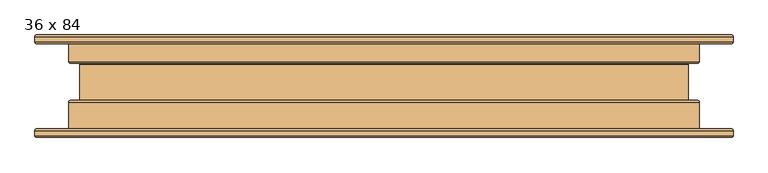
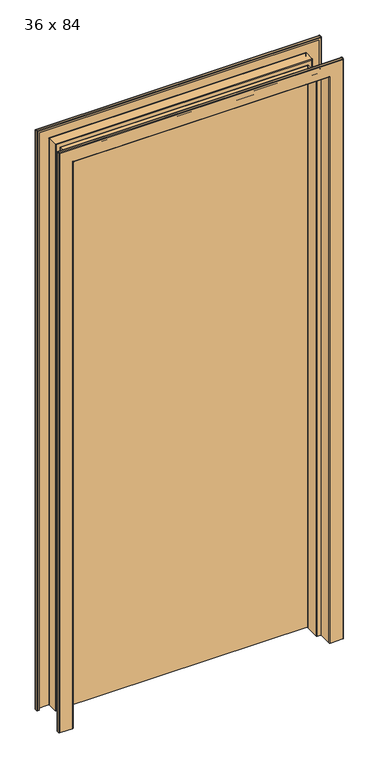
"""IFC4 building model written with IfcOpenShell, lengths in millimetres: door geometry, Door-Dunbarton_Doors-Hollow_Metal_Core : 36 x 84."""

from ifc_helpers import new_model, si_unit, frame, origin, origin_with_axes, place, context, project, spatial, polyline, circle_curve, ellipse_curve, outline, extrude, source, transform, mapped, element, save
from ifc_brep_helpers import plane_surface, cylinder_surface, revolved_surface, advanced_brep


def door_36_x_84_ee10bf19(model_context):
    return source(origin(), model_context, "Body", "SolidModel", [
        advanced_brep(
        [(-505.42825, -61.976, 0.0), (-500.0625, -61.976, 0.0), (-500.0625, -63.53175, 0.0), (-505.42825, -63.53175, 0.0), (-506.44425, -64.54775, 0.0), (-506.44425, -72.0725, 0.0), (-505.42825, -73.0885, 0.0), (-459.77175, -73.0885, 0.0), (-458.75575, -72.0725, 0.0), (-458.75575, -23.27275, 0.0), (-456.184, -20.701, 0.0), (-443.89675, -20.701, 0.0), (-442.88075, -19.685, 0.0), (-442.88075, 32.1056, 0.0), (-443.89675, 33.1216, 0.0), (-456.184, 33.1216, 0.0), (-458.75575, 35.69335, 0.0), (-458.75575, 72.009, 0.0), (-459.77175, 73.025, 0.0), (-505.42825, 73.025, 0.0), (-506.44425, 72.009, 0.0), (-506.44425, 64.48425, 0.0), (-505.42825, 63.46825, 0.0), (-500.0625, 63.46825, 0.0), (-500.0625, 61.9125, 0.0), (-505.42825, 61.9125, 0.0), (-508.0, 64.48425, 0.0), (-508.0, 72.009, 0.0), (-505.42825, 74.58075, 0.0), (-459.77175, 74.58075, 0.0), (-457.2, 72.009, 0.0), (-457.2, 35.69335, 0.0), (-456.184, 34.67735, 0.0), (-443.89675, 34.67735, 0.0), (-441.325, 32.1056, 0.0), (-441.325, -19.685, 0.0), (-443.89675, -22.25675, 0.0), (-456.184, -22.25675, 0.0), (-457.2, -23.27275, 0.0), (-457.2, -72.0725, 0.0), (-459.77175, -74.64425, 0.0), (-505.42825, -74.64425, 0.0), (-508.0, -72.0725, 0.0), (-508.0, -64.54775, 0.0), (-508.0, -64.54775, 2184.4), (-505.42825, -61.976, 2181.82825), (-508.0, -72.0725, 2184.4), (-505.42825, -74.64425, 2181.82825), (-459.77175, -74.64425, 2136.17175), (459.77175, -74.64425, 2136.17175), (459.77175, -74.64425, 0.0), (505.42825, -74.64425, 0.0), (505.42825, -74.64425, 2181.82825), (-457.2, -72.0725, 2133.6), (-457.2, -23.27275, 2133.6), (-456.184, -22.25675, 2132.584), (-443.89675, -22.25675, 2120.29675), (443.89675, -22.25675, 2120.29675), (443.89675, -22.25675, 0.0), (456.184, -22.25675, 0.0), (456.184, -22.25675, 2132.584), (-441.325, -19.685, 2117.725), (-441.325, 32.1056, 2117.725), (-443.89675, 34.67735, 2120.29675), (-456.184, 34.67735, 2132.584), (456.184, 34.67735, 2132.584), (456.184, 34.67735, 0.0), (443.89675, 34.67735, 0.0), (443.89675, 34.67735, 2120.29675), (-457.2, 35.69335, 2133.6), (-457.2, 72.009, 2133.6), (-459.77175, 74.58075, 2136.17175), (-505.42825, 74.58075, 2181.82825), (505.42825, 74.58075, 2181.82825), (505.42825, 74.58075, 0.0), (459.77175, 74.58075, 0.0), (459.77175, 74.58075, 2136.17175), (-508.0, 72.009, 2184.4), (-508.0, 64.48425, 2184.4), (-505.42825, 61.9125, 2181.82825), (-500.0625, 61.9125, 2176.4625), (500.0625, 61.9125, 2176.4625), (500.0625, 61.9125, 0.0), (505.42825, 61.9125, 0.0), (505.42825, 61.9125, 2181.82825), (-500.0625, 63.46825, 2176.4625), (-505.42825, 63.46825, 2181.82825), (505.42825, 63.46825, 2181.82825), (505.42825, 63.46825, 0.0), (500.0625, 63.46825, 0.0), (500.0625, 63.46825, 2176.4625), (-506.44425, 64.48425, 2182.84425), (-506.44425, 72.009, 2182.84425), (-505.42825, 73.025, 2181.82825), (-459.77175, 73.025, 2136.17175), (459.77175, 73.025, 2136.17175), (459.77175, 73.025, 0.0), (505.42825, 73.025, 0.0), (505.42825, 73.025, 2181.82825), (-458.75575, 72.009, 2135.15575), (-458.75575, 35.69335, 2135.15575), (-456.184, 33.1216, 2132.584), (-443.89675, 33.1216, 2120.29675), (443.89675, 33.1216, 2120.29675), (443.89675, 33.1216, 0.0), (456.184, 33.1216, 0.0), (456.184, 33.1216, 2132.584), (-442.88075, 32.1056, 2119.28075), (-442.88075, -19.685, 2119.28075), (-443.89675, -20.701, 2120.29675), (-456.184, -20.701, 2132.584), (456.184, -20.701, 2132.584), (456.184, -20.701, 0.0), (443.89675, -20.701, 0.0), (443.89675, -20.701, 2120.29675), (-458.75575, -23.27275, 2135.15575), (-458.75575, -72.0725, 2135.15575), (-459.77175, -73.0885, 2136.17175), (-505.42825, -73.0885, 2181.82825), (505.42825, -73.0885, 2181.82825), (505.42825, -73.0885, 0.0), (459.77175, -73.0885, 0.0), (459.77175, -73.0885, 2136.17175), (-506.44425, -72.0725, 2182.84425), (-506.44425, -64.54775, 2182.84425), (-505.42825, -63.53175, 2181.82825), (-500.0625, -63.53175, 2176.4625), (500.0625, -63.53175, 2176.4625), (500.0625, -63.53175, 0.0), (505.42825, -63.53175, 0.0), (505.42825, -63.53175, 2181.82825), (-500.0625, -61.976, 2176.4625), (505.42825, -61.976, 2181.82825), (505.42825, -61.976, 0.0), (500.0625, -61.976, 0.0), (500.0625, -61.976, 2176.4625), (508.0, -64.54775, 2184.4), (508.0, -72.0725, 2184.4), (457.2, -72.0725, 2133.6), (457.2, -23.27275, 2133.6), (441.325, -19.685, 2117.725), (441.325, 32.1056, 2117.725), (457.2, 35.69335, 2133.6), (457.2, 72.009, 2133.6), (508.0, 72.009, 2184.4), (508.0, 64.48425, 2184.4), (506.44425, 64.48425, 2182.84425), (506.44425, 72.009, 2182.84425), (458.75575, 72.009, 2135.15575), (458.75575, 35.69335, 2135.15575), (442.88075, 32.1056, 2119.28075), (442.88075, -19.685, 2119.28075), (458.75575, -23.27275, 2135.15575), (458.75575, -72.0725, 2135.15575), (506.44425, -72.0725, 2182.84425), (506.44425, -64.54775, 2182.84425), (508.0, -64.54775, 0.0), (508.0, -72.0725, 0.0), (457.2, -72.0725, 0.0), (457.2, -23.27275, 0.0), (441.325, -19.685, 0.0), (441.325, 32.1056, 0.0), (457.2, 35.69335, 0.0), (457.2, 72.009, 0.0), (508.0, 72.009, 0.0), (508.0, 64.48425, 0.0), (506.44425, 64.48425, 0.0), (506.44425, 72.009, 0.0), (458.75575, 72.009, 0.0), (458.75575, 35.69335, 0.0), (442.88075, 32.1056, 0.0), (442.88075, -19.685, 0.0), (458.75575, -23.27275, 0.0), (458.75575, -72.0725, 0.0), (506.44425, -72.0725, 0.0), (506.44425, -64.54775, 0.0)],
        [
            (0, 1),
            (1, 2),
            (2, 3),
            (3, 4, circle_curve(frame((-505.42825, -64.54775, 0.0), z_axis=(0.0, 0.0, 1.0), x_axis=(0.0, 1.0, 0.0)), 1.016)),
            (4, 5),
            (5, 6, circle_curve(frame((-505.42825, -72.0725, 0.0), z_axis=(0.0, 0.0, 1.0), x_axis=(0.0, 1.0, 0.0)), 1.016)),
            (6, 7),
            (7, 8, circle_curve(frame((-459.77175, -72.0725, 0.0), z_axis=(0.0, 0.0, 1.0), x_axis=(0.0, 1.0, 0.0)), 1.016)),
            (8, 9),
            (9, 10, circle_curve(frame((-456.184, -23.27275, 0.0), z_axis=(0.0, 0.0, -1.0), x_axis=(0.0, 1.0, 0.0)), 2.57175)),
            (10, 11),
            (11, 12, circle_curve(frame((-443.89675, -19.685, 0.0), z_axis=(0.0, 0.0, 1.0), x_axis=(0.0, 1.0, 0.0)), 1.016)),
            (12, 13),
            (13, 14, circle_curve(frame((-443.89675, 32.1056, 0.0), z_axis=(0.0, 0.0, 1.0), x_axis=(0.0, 1.0, 0.0)), 1.016)),
            (14, 15),
            (15, 16, circle_curve(frame((-456.184, 35.69335, 0.0), z_axis=(0.0, 0.0, -1.0), x_axis=(0.0, 1.0, 0.0)), 2.57175)),
            (16, 17),
            (17, 18, circle_curve(frame((-459.77175, 72.009, 0.0), z_axis=(0.0, 0.0, 1.0), x_axis=(0.0, 1.0, 0.0)), 1.016)),
            (18, 19),
            (19, 20, circle_curve(frame((-505.42825, 72.009, 0.0), z_axis=(0.0, 0.0, 1.0), x_axis=(0.0, 1.0, 0.0)), 1.016)),
            (20, 21),
            (21, 22, circle_curve(frame((-505.42825, 64.48425, 0.0), z_axis=(0.0, 0.0, 1.0), x_axis=(0.0, 1.0, 0.0)), 1.016)),
            (22, 23),
            (23, 24),
            (24, 25),
            (25, 26, circle_curve(frame((-505.42825, 64.48425, 0.0), z_axis=(0.0, 0.0, -1.0), x_axis=(0.0, 1.0, 0.0)), 2.57175)),
            (26, 27),
            (27, 28, circle_curve(frame((-505.42825, 72.009, 0.0), z_axis=(0.0, 0.0, -1.0), x_axis=(0.0, 1.0, 0.0)), 2.57175)),
            (28, 29),
            (29, 30, circle_curve(frame((-459.77175, 72.009, 0.0), z_axis=(0.0, 0.0, -1.0), x_axis=(0.0, 1.0, 0.0)), 2.57175)),
            (30, 31),
            (31, 32, circle_curve(frame((-456.184, 35.69335, 0.0), z_axis=(0.0, 0.0, 1.0), x_axis=(0.0, 1.0, 0.0)), 1.016)),
            (32, 33),
            (33, 34, circle_curve(frame((-443.89675, 32.1056, 0.0), z_axis=(0.0, 0.0, -1.0), x_axis=(0.0, 1.0, 0.0)), 2.57175)),
            (34, 35),
            (35, 36, circle_curve(frame((-443.89675, -19.685, 0.0), z_axis=(0.0, 0.0, -1.0), x_axis=(0.0, 1.0, 0.0)), 2.57175)),
            (36, 37),
            (37, 38, circle_curve(frame((-456.184, -23.27275, 0.0), z_axis=(0.0, 0.0, 1.0), x_axis=(0.0, 1.0, 0.0)), 1.016)),
            (38, 39),
            (39, 40, circle_curve(frame((-459.77175, -72.0725, 0.0), z_axis=(0.0, 0.0, -1.0), x_axis=(0.0, 1.0, 0.0)), 2.57175)),
            (40, 41),
            (41, 42, circle_curve(frame((-505.42825, -72.0725, 0.0), z_axis=(0.0, 0.0, -1.0), x_axis=(0.0, 1.0, 0.0)), 2.57175)),
            (42, 43),
            (43, 0, circle_curve(frame((-505.42825, -64.54775, 0.0), z_axis=(0.0, 0.0, -1.0), x_axis=(0.0, 1.0, 0.0)), 2.57175)),
            (43, 44),
            (44, 45, ellipse_curve(frame((-505.42825, -64.54775, 2181.82825), z_axis=(-0.7071067811865475, 0.0, -0.7071067811865475), x_axis=(0.7071067811865474, 0.0, -0.7071067811865476)), 3.6370037, 2.57175)),
            (45, 0),
            (42, 46),
            (46, 44),
            (41, 47),
            (47, 46, ellipse_curve(frame((-505.42825, -72.0725, 2181.82825), z_axis=(-0.7071067811865475, 0.0, -0.7071067811865475), x_axis=(0.7071067811865474, 0.0, -0.7071067811865476)), 3.6370037, 2.57175)),
            (40, 48),
            (48, 49),
            (49, 50),
            (50, 51),
            (51, 52),
            (52, 47),
            (39, 53),
            (53, 48, ellipse_curve(frame((-459.77175, -72.0725, 2136.17175), z_axis=(-0.7071067811865475, 0.0, -0.7071067811865475), x_axis=(0.7071067811865474, 0.0, -0.7071067811865476)), 3.6370037, 2.57175)),
            (38, 54),
            (54, 53),
            (37, 55),
            (55, 54, ellipse_curve(frame((-456.184, -23.27275, 2132.584), z_axis=(0.7071067811865475, 0.0, 0.7071067811865475), x_axis=(-0.7071067811865474, 0.0, 0.7071067811865476)), 1.436841, 1.016)),
            (36, 56),
            (56, 57),
            (57, 58),
            (58, 59),
            (59, 60),
            (60, 55),
            (35, 61),
            (61, 56, ellipse_curve(frame((-443.89675, -19.685, 2120.29675), z_axis=(-0.7071067811865475, 0.0, -0.7071067811865475), x_axis=(0.7071067811865474, 0.0, -0.7071067811865476)), 3.6370037, 2.57175)),
            (34, 62),
            (62, 61),
            (33, 63),
            (63, 62, ellipse_curve(frame((-443.89675, 32.1056, 2120.29675), z_axis=(-0.7071067811865475, 0.0, -0.7071067811865475), x_axis=(0.7071067811865474, 0.0, -0.7071067811865476)), 3.6370037, 2.57175)),
            (32, 64),
            (64, 65),
            (65, 66),
            (66, 67),
            (67, 68),
            (68, 63),
            (31, 69),
            (69, 64, ellipse_curve(frame((-456.184, 35.69335, 2132.584), z_axis=(0.7071067811865475, 0.0, 0.7071067811865475), x_axis=(-0.7071067811865474, 0.0, 0.7071067811865476)), 1.436841, 1.016)),
            (30, 70),
            (70, 69),
            (29, 71),
            (71, 70, ellipse_curve(frame((-459.77175, 72.009, 2136.17175), z_axis=(-0.7071067811865475, 0.0, -0.7071067811865475), x_axis=(0.7071067811865474, 0.0, -0.7071067811865476)), 3.6370037, 2.57175)),
            (28, 72),
            (72, 73),
            (73, 74),
            (74, 75),
            (75, 76),
            (76, 71),
            (27, 77),
            (77, 72, ellipse_curve(frame((-505.42825, 72.009, 2181.82825), z_axis=(-0.7071067811865475, 0.0, -0.7071067811865475), x_axis=(0.7071067811865474, 0.0, -0.7071067811865476)), 3.6370037, 2.57175)),
            (26, 78),
            (78, 77),
            (25, 79),
            (79, 78, ellipse_curve(frame((-505.42825, 64.48425, 2181.82825), z_axis=(-0.7071067811865475, 0.0, -0.7071067811865475), x_axis=(0.7071067811865474, 0.0, -0.7071067811865476)), 3.6370037, 2.57175)),
            (24, 80),
            (80, 81),
            (81, 82),
            (82, 83),
            (83, 84),
            (84, 79),
            (23, 85),
            (85, 80),
            (22, 86),
            (86, 87),
            (87, 88),
            (88, 89),
            (89, 90),
            (90, 85),
            (21, 91),
            (91, 86, ellipse_curve(frame((-505.42825, 64.48425, 2181.82825), z_axis=(0.7071067811865475, 0.0, 0.7071067811865475), x_axis=(-0.7071067811865474, 0.0, 0.7071067811865476)), 1.436841, 1.016)),
            (20, 92),
            (92, 91),
            (19, 93),
            (93, 92, ellipse_curve(frame((-505.42825, 72.009, 2181.82825), z_axis=(0.7071067811865475, 0.0, 0.7071067811865475), x_axis=(-0.7071067811865474, 0.0, 0.7071067811865476)), 1.436841, 1.016)),
            (18, 94),
            (94, 95),
            (95, 96),
            (96, 97),
            (97, 98),
            (98, 93),
            (17, 99),
            (99, 94, ellipse_curve(frame((-459.77175, 72.009, 2136.17175), z_axis=(0.7071067811865475, 0.0, 0.7071067811865475), x_axis=(-0.7071067811865474, 0.0, 0.7071067811865476)), 1.436841, 1.016)),
            (16, 100),
            (100, 99),
            (15, 101),
            (101, 100, ellipse_curve(frame((-456.184, 35.69335, 2132.584), z_axis=(-0.7071067811865475, 0.0, -0.7071067811865475), x_axis=(0.7071067811865474, 0.0, -0.7071067811865476)), 3.6370037, 2.57175)),
            (14, 102),
            (102, 103),
            (103, 104),
            (104, 105),
            (105, 106),
            (106, 101),
            (13, 107),
            (107, 102, ellipse_curve(frame((-443.89675, 32.1056, 2120.29675), z_axis=(0.7071067811865475, 0.0, 0.7071067811865475), x_axis=(-0.7071067811865474, 0.0, 0.7071067811865476)), 1.436841, 1.016)),
            (12, 108),
            (108, 107),
            (11, 109),
            (109, 108, ellipse_curve(frame((-443.89675, -19.685, 2120.29675), z_axis=(0.7071067811865475, 0.0, 0.7071067811865475), x_axis=(-0.7071067811865474, 0.0, 0.7071067811865476)), 1.436841, 1.016)),
            (10, 110),
            (110, 111),
            (111, 112),
            (112, 113),
            (113, 114),
            (114, 109),
            (9, 115),
            (115, 110, ellipse_curve(frame((-456.184, -23.27275, 2132.584), z_axis=(-0.7071067811865475, 0.0, -0.7071067811865475), x_axis=(0.7071067811865474, 0.0, -0.7071067811865476)), 3.6370037, 2.57175)),
            (8, 116),
            (116, 115),
            (7, 117),
            (117, 116, ellipse_curve(frame((-459.77175, -72.0725, 2136.17175), z_axis=(0.7071067811865475, 0.0, 0.7071067811865475), x_axis=(-0.7071067811865474, 0.0, 0.7071067811865476)), 1.436841, 1.016)),
            (6, 118),
            (118, 119),
            (119, 120),
            (120, 121),
            (121, 122),
            (122, 117),
            (5, 123),
            (123, 118, ellipse_curve(frame((-505.42825, -72.0725, 2181.82825), z_axis=(0.7071067811865475, 0.0, 0.7071067811865475), x_axis=(-0.7071067811865474, 0.0, 0.7071067811865476)), 1.436841, 1.016)),
            (4, 124),
            (124, 123),
            (3, 125),
            (125, 124, ellipse_curve(frame((-505.42825, -64.54775, 2181.82825), z_axis=(0.7071067811865475, 0.0, 0.7071067811865475), x_axis=(-0.7071067811865474, 0.0, 0.7071067811865476)), 1.436841, 1.016)),
            (2, 126),
            (126, 127),
            (127, 128),
            (128, 129),
            (129, 130),
            (130, 125),
            (1, 131),
            (131, 126),
            (45, 132),
            (132, 133),
            (133, 134),
            (134, 135),
            (135, 131),
            (44, 136),
            (136, 132, ellipse_curve(frame((505.42825, -64.54775, 2181.82825), z_axis=(-0.7071067811865475, 0.0, 0.7071067811865475), x_axis=(-0.7071067811865476, 0.0, -0.7071067811865474)), 3.6370037, 2.57175)),
            (46, 137),
            (137, 136),
            (52, 137, ellipse_curve(frame((505.42825, -72.0725, 2181.82825), z_axis=(-0.7071067811865475, 0.0, 0.7071067811865475), x_axis=(-0.7071067811865476, 0.0, -0.7071067811865474)), 3.6370037, 2.57175)),
            (53, 138),
            (138, 49, ellipse_curve(frame((459.77175, -72.0725, 2136.17175), z_axis=(-0.7071067811865475, 0.0, 0.7071067811865475), x_axis=(-0.7071067811865476, 0.0, -0.7071067811865474)), 3.6370037, 2.57175)),
            (54, 139),
            (139, 138),
            (60, 139, ellipse_curve(frame((456.184, -23.27275, 2132.584), z_axis=(0.7071067811865475, 0.0, -0.7071067811865475), x_axis=(0.7071067811865476, 0.0, 0.7071067811865474)), 1.436841, 1.016)),
            (61, 140),
            (140, 57, ellipse_curve(frame((443.89675, -19.685, 2120.29675), z_axis=(-0.7071067811865475, 0.0, 0.7071067811865475), x_axis=(-0.7071067811865476, 0.0, -0.7071067811865474)), 3.6370037, 2.57175)),
            (62, 141),
            (141, 140),
            (68, 141, ellipse_curve(frame((443.89675, 32.1056, 2120.29675), z_axis=(-0.7071067811865475, 0.0, 0.7071067811865475), x_axis=(-0.7071067811865476, 0.0, -0.7071067811865474)), 3.6370037, 2.57175)),
            (69, 142),
            (142, 65, ellipse_curve(frame((456.184, 35.69335, 2132.584), z_axis=(0.7071067811865475, 0.0, -0.7071067811865475), x_axis=(0.7071067811865476, 0.0, 0.7071067811865474)), 1.436841, 1.016)),
            (70, 143),
            (143, 142),
            (76, 143, ellipse_curve(frame((459.77175, 72.009, 2136.17175), z_axis=(-0.7071067811865475, 0.0, 0.7071067811865475), x_axis=(-0.7071067811865476, 0.0, -0.7071067811865474)), 3.6370037, 2.57175)),
            (77, 144),
            (144, 73, ellipse_curve(frame((505.42825, 72.009, 2181.82825), z_axis=(-0.7071067811865475, 0.0, 0.7071067811865475), x_axis=(-0.7071067811865476, 0.0, -0.7071067811865474)), 3.6370037, 2.57175)),
            (78, 145),
            (145, 144),
            (84, 145, ellipse_curve(frame((505.42825, 64.48425, 2181.82825), z_axis=(-0.7071067811865475, 0.0, 0.7071067811865475), x_axis=(-0.7071067811865476, 0.0, -0.7071067811865474)), 3.6370037, 2.57175)),
            (90, 81),
            (91, 146),
            (146, 87, ellipse_curve(frame((505.42825, 64.48425, 2181.82825), z_axis=(0.7071067811865475, 0.0, -0.7071067811865475), x_axis=(0.7071067811865476, 0.0, 0.7071067811865474)), 1.436841, 1.016)),
            (92, 147),
            (147, 146),
            (98, 147, ellipse_curve(frame((505.42825, 72.009, 2181.82825), z_axis=(0.7071067811865475, 0.0, -0.7071067811865475), x_axis=(0.7071067811865476, 0.0, 0.7071067811865474)), 1.436841, 1.016)),
            (99, 148),
            (148, 95, ellipse_curve(frame((459.77175, 72.009, 2136.17175), z_axis=(0.7071067811865475, 0.0, -0.7071067811865475), x_axis=(0.7071067811865476, 0.0, 0.7071067811865474)), 1.436841, 1.016)),
            (100, 149),
            (149, 148),
            (106, 149, ellipse_curve(frame((456.184, 35.69335, 2132.584), z_axis=(-0.7071067811865475, 0.0, 0.7071067811865475), x_axis=(-0.7071067811865476, 0.0, -0.7071067811865474)), 3.6370037, 2.57175)),
            (107, 150),
            (150, 103, ellipse_curve(frame((443.89675, 32.1056, 2120.29675), z_axis=(0.7071067811865475, 0.0, -0.7071067811865475), x_axis=(0.7071067811865476, 0.0, 0.7071067811865474)), 1.436841, 1.016)),
            (108, 151),
            (151, 150),
            (114, 151, ellipse_curve(frame((443.89675, -19.685, 2120.29675), z_axis=(0.7071067811865475, 0.0, -0.7071067811865475), x_axis=(0.7071067811865476, 0.0, 0.7071067811865474)), 1.436841, 1.016)),
            (115, 152),
            (152, 111, ellipse_curve(frame((456.184, -23.27275, 2132.584), z_axis=(-0.7071067811865475, 0.0, 0.7071067811865475), x_axis=(-0.7071067811865476, 0.0, -0.7071067811865474)), 3.6370037, 2.57175)),
            (116, 153),
            (153, 152),
            (122, 153, ellipse_curve(frame((459.77175, -72.0725, 2136.17175), z_axis=(0.7071067811865475, 0.0, -0.7071067811865475), x_axis=(0.7071067811865476, 0.0, 0.7071067811865474)), 1.436841, 1.016)),
            (123, 154),
            (154, 119, ellipse_curve(frame((505.42825, -72.0725, 2181.82825), z_axis=(0.7071067811865475, 0.0, -0.7071067811865475), x_axis=(0.7071067811865476, 0.0, 0.7071067811865474)), 1.436841, 1.016)),
            (124, 155),
            (155, 154),
            (130, 155, ellipse_curve(frame((505.42825, -64.54775, 2181.82825), z_axis=(0.7071067811865475, 0.0, -0.7071067811865475), x_axis=(0.7071067811865476, 0.0, 0.7071067811865474)), 1.436841, 1.016)),
            (135, 127),
            (133, 156, circle_curve(frame((505.42825, -64.54775, 0.0), z_axis=(0.0, 0.0, -1.0), x_axis=(0.0, 1.0, 0.0)), 2.57175)),
            (156, 157),
            (157, 51, circle_curve(frame((505.42825, -72.0725, 0.0), z_axis=(0.0, 0.0, -1.0), x_axis=(0.0, 1.0, 0.0)), 2.57175)),
            (50, 158, circle_curve(frame((459.77175, -72.0725, 0.0), z_axis=(0.0, 0.0, -1.0), x_axis=(0.0, 1.0, 0.0)), 2.57175)),
            (158, 159),
            (159, 59, circle_curve(frame((456.184, -23.27275, 0.0), z_axis=(0.0, 0.0, 1.0), x_axis=(0.0, 1.0, 0.0)), 1.016)),
            (58, 160, circle_curve(frame((443.89675, -19.685, 0.0), z_axis=(0.0, 0.0, -1.0), x_axis=(0.0, 1.0, 0.0)), 2.57175)),
            (160, 161),
            (161, 67, circle_curve(frame((443.89675, 32.1056, 0.0), z_axis=(0.0, 0.0, -1.0), x_axis=(0.0, 1.0, 0.0)), 2.57175)),
            (66, 162, circle_curve(frame((456.184, 35.69335, 0.0), z_axis=(0.0, 0.0, 1.0), x_axis=(0.0, 1.0, 0.0)), 1.016)),
            (162, 163),
            (163, 75, circle_curve(frame((459.77175, 72.009, 0.0), z_axis=(0.0, 0.0, -1.0), x_axis=(0.0, 1.0, 0.0)), 2.57175)),
            (74, 164, circle_curve(frame((505.42825, 72.009, 0.0), z_axis=(0.0, 0.0, -1.0), x_axis=(0.0, 1.0, 0.0)), 2.57175)),
            (164, 165),
            (165, 83, circle_curve(frame((505.42825, 64.48425, 0.0), z_axis=(0.0, 0.0, -1.0), x_axis=(0.0, 1.0, 0.0)), 2.57175)),
            (82, 89),
            (88, 166, circle_curve(frame((505.42825, 64.48425, 0.0), z_axis=(0.0, 0.0, 1.0), x_axis=(0.0, 1.0, 0.0)), 1.016)),
            (166, 167),
            (167, 97, circle_curve(frame((505.42825, 72.009, 0.0), z_axis=(0.0, 0.0, 1.0), x_axis=(0.0, 1.0, 0.0)), 1.016)),
            (96, 168, circle_curve(frame((459.77175, 72.009, 0.0), z_axis=(0.0, 0.0, 1.0), x_axis=(0.0, 1.0, 0.0)), 1.016)),
            (168, 169),
            (169, 105, circle_curve(frame((456.184, 35.69335, 0.0), z_axis=(0.0, 0.0, -1.0), x_axis=(0.0, 1.0, 0.0)), 2.57175)),
            (104, 170, circle_curve(frame((443.89675, 32.1056, 0.0), z_axis=(0.0, 0.0, 1.0), x_axis=(0.0, 1.0, 0.0)), 1.016)),
            (170, 171),
            (171, 113, circle_curve(frame((443.89675, -19.685, 0.0), z_axis=(0.0, 0.0, 1.0), x_axis=(0.0, 1.0, 0.0)), 1.016)),
            (112, 172, circle_curve(frame((456.184, -23.27275, 0.0), z_axis=(0.0, 0.0, -1.0), x_axis=(0.0, 1.0, 0.0)), 2.57175)),
            (172, 173),
            (173, 121, circle_curve(frame((459.77175, -72.0725, 0.0), z_axis=(0.0, 0.0, 1.0), x_axis=(0.0, 1.0, 0.0)), 1.016)),
            (120, 174, circle_curve(frame((505.42825, -72.0725, 0.0), z_axis=(0.0, 0.0, 1.0), x_axis=(0.0, 1.0, 0.0)), 1.016)),
            (174, 175),
            (175, 129, circle_curve(frame((505.42825, -64.54775, 0.0), z_axis=(0.0, 0.0, 1.0), x_axis=(0.0, 1.0, 0.0)), 1.016)),
            (128, 134),
            (136, 156),
            (137, 157),
            (138, 158),
            (139, 159),
            (140, 160),
            (141, 161),
            (142, 162),
            (143, 163),
            (144, 164),
            (145, 165),
            (146, 166),
            (147, 167),
            (148, 168),
            (149, 169),
            (150, 170),
            (151, 171),
            (152, 172),
            (153, 173),
            (154, 174),
            (155, 175),
        ],
        [
            plane_surface(frame((-468.3125, 61.9125, 0.0), z_axis=(0.0, 0.0, -1.0), x_axis=(1.0, 0.0, 0.0))),
            cylinder_surface(frame((-505.42825, -64.54775, 0.0), z_axis=(0.0, 0.0, -1.0), x_axis=(0.0, 1.0, 0.0)), 2.57175),
            plane_surface(frame((-508.0, -64.54775, 0.0), z_axis=(-1.0, 0.0, 0.0), x_axis=(0.0, 0.0, 1.0))),
            cylinder_surface(frame((-505.42825, -72.0725, 0.0), z_axis=(0.0, 0.0, -1.0), x_axis=(0.0, 1.0, 0.0)), 2.57175),
            plane_surface(frame((-505.42825, -74.64425, 0.0), z_axis=(0.0, -1.0, 0.0), x_axis=(0.0, 0.0, 1.0))),
            cylinder_surface(frame((-459.77175, -72.0725, 0.0), z_axis=(0.0, 0.0, -1.0), x_axis=(0.0, 1.0, 0.0)), 2.57175),
            plane_surface(frame((-457.2, -72.0725, 0.0), z_axis=(1.0, 0.0, 0.0), x_axis=(0.0, 0.0, 1.0))),
            revolved_surface(polyline([(-456.184, -22.256749999999997, 2133.600000014587), (-456.184, -22.256749999999997, 0.0)]), (-456.184, -23.27275, 0.0), (0.0, 0.0, 1.0)),
            plane_surface(frame((-456.184, -22.25675, 0.0), z_axis=(0.0, -1.0, 0.0), x_axis=(0.0, 0.0, 1.0))),
            cylinder_surface(frame((-443.89675, -19.685, 0.0), z_axis=(0.0, 0.0, -1.0), x_axis=(0.0, 1.0, 0.0)), 2.57175),
            plane_surface(frame((-441.325, -19.685, 0.0), z_axis=(1.0, 0.0, 0.0), x_axis=(0.0, 0.0, 1.0))),
            cylinder_surface(frame((-443.89675, 32.1056, 0.0), z_axis=(0.0, 0.0, -1.0), x_axis=(0.0, 1.0, 0.0)), 2.57175),
            plane_surface(frame((-443.89675, 34.67735, 0.0), z_axis=(0.0, 1.0, 0.0), x_axis=(0.0, 0.0, 1.0))),
            revolved_surface(polyline([(-456.184, 36.70935, 2133.600000014587), (-456.184, 36.70935, 0.0)]), (-456.184, 35.69335, 0.0), (0.0, 0.0, 1.0)),
            plane_surface(frame((-457.2, 35.69335, 0.0), z_axis=(1.0, 0.0, 0.0), x_axis=(0.0, 0.0, 1.0))),
            cylinder_surface(frame((-459.77175, 72.009, 0.0), z_axis=(0.0, 0.0, -1.0), x_axis=(0.0, 1.0, 0.0)), 2.57175),
            plane_surface(frame((-459.77175, 74.58075, 0.0), z_axis=(0.0, 1.0, 0.0), x_axis=(0.0, 0.0, 1.0))),
            cylinder_surface(frame((-505.42825, 72.009, 0.0), z_axis=(0.0, 0.0, -1.0), x_axis=(0.0, 1.0, 0.0)), 2.57175),
            plane_surface(frame((-508.0, 72.009, 0.0), z_axis=(-1.0, 0.0, 0.0), x_axis=(0.0, 0.0, 1.0))),
            cylinder_surface(frame((-505.42825, 64.48425, 0.0), z_axis=(0.0, 0.0, -1.0), x_axis=(0.0, 1.0, 0.0)), 2.57175),
            plane_surface(frame((-505.42825, 61.9125, 0.0), z_axis=(0.0, -1.0, 0.0), x_axis=(0.0, 0.0, 1.0))),
            plane_surface(frame((-500.0625, 61.9125, 0.0), z_axis=(1.0, 0.0, 0.0), x_axis=(0.0, 0.0, 1.0))),
            plane_surface(frame((-500.0625, 63.46825, 0.0), z_axis=(0.0, 1.0, 0.0), x_axis=(0.0, 0.0, 1.0))),
            revolved_surface(polyline([(-505.42825, 65.50025000000001, 2182.844250014587), (-505.42825, 65.50025000000001, 0.0)]), (-505.42825, 64.48425, 0.0), (0.0, 0.0, 1.0)),
            plane_surface(frame((-506.44425, 64.48425, 0.0), z_axis=(1.0, 0.0, 0.0), x_axis=(0.0, 0.0, 1.0))),
            revolved_surface(polyline([(-505.42825, 73.025, 2182.844250014587), (-505.42825, 73.025, 0.0)]), (-505.42825, 72.009, 0.0), (0.0, 0.0, 1.0)),
            plane_surface(frame((-505.42825, 73.025, 0.0), z_axis=(0.0, -1.0, 0.0), x_axis=(0.0, 0.0, 1.0))),
            revolved_surface(polyline([(-459.77175, 73.025, 2137.187750014587), (-459.77175, 73.025, 0.0)]), (-459.77175, 72.009, 0.0), (0.0, 0.0, 1.0)),
            plane_surface(frame((-458.75575, 72.009, 0.0), z_axis=(-1.0, 0.0, 0.0), x_axis=(0.0, 0.0, 1.0))),
            cylinder_surface(frame((-456.184, 35.69335, 0.0), z_axis=(0.0, 0.0, -1.0), x_axis=(0.0, 1.0, 0.0)), 2.57175),
            plane_surface(frame((-456.184, 33.1216, 0.0), z_axis=(0.0, -1.0, 0.0), x_axis=(0.0, 0.0, 1.0))),
            revolved_surface(polyline([(-443.89675, 33.1216, 2121.312750014587), (-443.89675, 33.1216, 0.0)]), (-443.89675, 32.1056, 0.0), (0.0, 0.0, 1.0)),
            plane_surface(frame((-442.88075, 32.1056, 0.0), z_axis=(-1.0, 0.0, 0.0), x_axis=(0.0, 0.0, 1.0))),
            revolved_surface(polyline([(-443.89675, -18.668999999999997, 2121.312750014587), (-443.89675, -18.668999999999997, 0.0)]), (-443.89675, -19.685, 0.0), (0.0, 0.0, 1.0)),
            plane_surface(frame((-443.89675, -20.701, 0.0), z_axis=(0.0, 1.0, 0.0), x_axis=(0.0, 0.0, 1.0))),
            cylinder_surface(frame((-456.184, -23.27275, 0.0), z_axis=(0.0, 0.0, -1.0), x_axis=(0.0, 1.0, 0.0)), 2.57175),
            plane_surface(frame((-458.75575, -23.27275, 0.0), z_axis=(-1.0, 0.0, 0.0), x_axis=(0.0, 0.0, 1.0))),
            revolved_surface(polyline([(-459.77175, -71.0565, 2137.187750014587), (-459.77175, -71.0565, 0.0)]), (-459.77175, -72.0725, 0.0), (0.0, 0.0, 1.0)),
            plane_surface(frame((-459.77175, -73.0885, 0.0), z_axis=(0.0, 1.0, 0.0), x_axis=(0.0, 0.0, 1.0))),
            revolved_surface(polyline([(-505.42825, -71.0565, 2182.844250014587), (-505.42825, -71.0565, 0.0)]), (-505.42825, -72.0725, 0.0), (0.0, 0.0, 1.0)),
            plane_surface(frame((-506.44425, -72.0725, 0.0), z_axis=(1.0, 0.0, 0.0), x_axis=(0.0, 0.0, 1.0))),
            revolved_surface(polyline([(-505.42825, -63.531749999999995, 2182.844250014587), (-505.42825, -63.531749999999995, 0.0)]), (-505.42825, -64.54775, 0.0), (0.0, 0.0, 1.0)),
            plane_surface(frame((-505.42825, -63.53175, 0.0), z_axis=(0.0, -1.0, 0.0), x_axis=(0.0, 0.0, 1.0))),
            plane_surface(frame((-500.0625, -63.53175, 0.0), z_axis=(1.0, 0.0, 0.0), x_axis=(0.0, 0.0, 1.0))),
            plane_surface(frame((-500.0625, -61.976, 0.0), z_axis=(0.0, 1.0, 0.0), x_axis=(0.0, 0.0, 1.0))),
            cylinder_surface(frame((-468.3125, -64.54775, 2181.82825), z_axis=(-1.0, 0.0, 0.0), x_axis=(0.0, 1.0, 0.0)), 2.57175),
            plane_surface(frame((-508.0, -64.54775, 2184.4), z_axis=(0.0, 0.0, 1.0), x_axis=(1.0, 0.0, 0.0))),
            cylinder_surface(frame((-468.3125, -72.0725, 2181.82825), z_axis=(-1.0, 0.0, 0.0), x_axis=(0.0, 1.0, 0.0)), 2.57175),
            cylinder_surface(frame((-468.3125, -72.0725, 2136.17175), z_axis=(-1.0, 0.0, 0.0), x_axis=(0.0, 1.0, 0.0)), 2.57175),
            plane_surface(frame((-457.2, -72.0725, 2133.6), z_axis=(0.0, 0.0, -1.0), x_axis=(1.0, 0.0, 0.0))),
            revolved_surface(polyline([(457.20000001458686, -22.256749999999997, 2132.584), (-457.20000001458686, -22.256749999999997, 2132.584)]), (-468.3125, -23.27275, 2132.584), (1.0, 0.0, 0.0)),
            cylinder_surface(frame((-468.3125, -19.685, 2120.29675), z_axis=(-1.0, 0.0, 0.0), x_axis=(0.0, 1.0, 0.0)), 2.57175),
            plane_surface(frame((-441.325, -19.685, 2117.725), z_axis=(0.0, 0.0, -1.0), x_axis=(1.0, 0.0, 0.0))),
            cylinder_surface(frame((-468.3125, 32.1056, 2120.29675), z_axis=(-1.0, 0.0, 0.0), x_axis=(0.0, 1.0, 0.0)), 2.57175),
            revolved_surface(polyline([(457.20000001458686, 36.70935, 2132.584), (-457.20000001458686, 36.70935, 2132.584)]), (-468.3125, 35.69335, 2132.584), (1.0, 0.0, 0.0)),
            plane_surface(frame((-457.2, 35.69335, 2133.6), z_axis=(0.0, 0.0, -1.0), x_axis=(1.0, 0.0, 0.0))),
            cylinder_surface(frame((-468.3125, 72.009, 2136.17175), z_axis=(-1.0, 0.0, 0.0), x_axis=(0.0, 1.0, 0.0)), 2.57175),
            cylinder_surface(frame((-468.3125, 72.009, 2181.82825), z_axis=(-1.0, 0.0, 0.0), x_axis=(0.0, 1.0, 0.0)), 2.57175),
            plane_surface(frame((-508.0, 72.009, 2184.4), z_axis=(0.0, 0.0, 1.0), x_axis=(1.0, 0.0, 0.0))),
            cylinder_surface(frame((-468.3125, 64.48425, 2181.82825), z_axis=(-1.0, 0.0, 0.0), x_axis=(0.0, 1.0, 0.0)), 2.57175),
            plane_surface(frame((-500.0625, 61.9125, 2176.4625), z_axis=(0.0, 0.0, -1.0), x_axis=(1.0, 0.0, 0.0))),
            revolved_surface(polyline([(506.4442500145868, 65.50025000000001, 2181.82825), (-506.4442500145868, 65.50025000000001, 2181.82825)]), (-468.3125, 64.48425, 2181.82825), (1.0, 0.0, 0.0)),
            plane_surface(frame((-506.44425, 64.48425, 2182.84425), z_axis=(0.0, 0.0, -1.0), x_axis=(1.0, 0.0, 0.0))),
            revolved_surface(polyline([(506.4442500145868, 73.025, 2181.82825), (-506.4442500145868, 73.025, 2181.82825)]), (-468.3125, 72.009, 2181.82825), (1.0, 0.0, 0.0)),
            revolved_surface(polyline([(460.7877500145869, 73.025, 2136.17175), (-460.78775001458683, 73.025, 2136.17175)]), (-468.3125, 72.009, 2136.17175), (1.0, 0.0, 0.0)),
            plane_surface(frame((-458.75575, 72.009, 2135.15575), z_axis=(0.0, 0.0, 1.0), x_axis=(1.0, 0.0, 0.0))),
            cylinder_surface(frame((-468.3125, 35.69335, 2132.584), z_axis=(-1.0, 0.0, 0.0), x_axis=(0.0, 1.0, 0.0)), 2.57175),
            revolved_surface(polyline([(444.9127500145869, 33.1216, 2120.29675), (-444.91275001458683, 33.1216, 2120.29675)]), (-468.3125, 32.1056, 2120.29675), (1.0, 0.0, 0.0)),
            plane_surface(frame((-442.88075, 32.1056, 2119.28075), z_axis=(0.0, 0.0, 1.0), x_axis=(1.0, 0.0, 0.0))),
            revolved_surface(polyline([(444.9127500145869, -18.668999999999997, 2120.29675), (-444.91275001458683, -18.668999999999997, 2120.29675)]), (-468.3125, -19.685, 2120.29675), (1.0, 0.0, 0.0)),
            cylinder_surface(frame((-468.3125, -23.27275, 2132.584), z_axis=(-1.0, 0.0, 0.0), x_axis=(0.0, 1.0, 0.0)), 2.57175),
            plane_surface(frame((-458.75575, -23.27275, 2135.15575), z_axis=(0.0, 0.0, 1.0), x_axis=(1.0, 0.0, 0.0))),
            revolved_surface(polyline([(460.7877500145869, -71.0565, 2136.17175), (-460.78775001458683, -71.0565, 2136.17175)]), (-468.3125, -72.0725, 2136.17175), (1.0, 0.0, 0.0)),
            revolved_surface(polyline([(506.4442500145868, -71.0565, 2181.82825), (-506.4442500145868, -71.0565, 2181.82825)]), (-468.3125, -72.0725, 2181.82825), (1.0, 0.0, 0.0)),
            plane_surface(frame((-506.44425, -72.0725, 2182.84425), z_axis=(0.0, 0.0, -1.0), x_axis=(1.0, 0.0, 0.0))),
            revolved_surface(polyline([(506.4442500145868, -63.531749999999995, 2181.82825), (-506.4442500145868, -63.531749999999995, 2181.82825)]), (-468.3125, -64.54775, 2181.82825), (1.0, 0.0, 0.0)),
            plane_surface(frame((-500.0625, -63.53175, 2176.4625), z_axis=(0.0, 0.0, -1.0), x_axis=(1.0, 0.0, 0.0))),
            plane_surface(frame((468.3125, 61.9125, 0.0), z_axis=(0.0, 0.0, -1.0), x_axis=(-1.0, 0.0, 0.0))),
            cylinder_surface(frame((505.42825, -64.54775, 2144.7125), z_axis=(0.0, 0.0, 1.0), x_axis=(0.0, 1.0, 0.0)), 2.57175),
            plane_surface(frame((508.0, -64.54775, 2184.4), z_axis=(1.0, 0.0, 0.0), x_axis=(0.0, 0.0, -1.0))),
            cylinder_surface(frame((505.42825, -72.0725, 2144.7125), z_axis=(0.0, 0.0, 1.0), x_axis=(0.0, 1.0, 0.0)), 2.57175),
            cylinder_surface(frame((459.77175, -72.0725, 2144.7125), z_axis=(0.0, 0.0, 1.0), x_axis=(0.0, 1.0, 0.0)), 2.57175),
            plane_surface(frame((457.2, -72.0725, 2133.6), z_axis=(-1.0, 0.0, 0.0), x_axis=(0.0, 0.0, -1.0))),
            revolved_surface(polyline([(456.184, -22.256749999999997, 0.0), (456.184, -22.256749999999997, 2133.600000014587)]), (456.184, -23.27275, 2144.7125), (0.0, 0.0, -1.0)),
            cylinder_surface(frame((443.89675, -19.685, 2144.7125), z_axis=(0.0, 0.0, 1.0), x_axis=(0.0, 1.0, 0.0)), 2.57175),
            plane_surface(frame((441.325, -19.685, 2117.725), z_axis=(-1.0, 0.0, 0.0), x_axis=(0.0, 0.0, -1.0))),
            cylinder_surface(frame((443.89675, 32.1056, 2144.7125), z_axis=(0.0, 0.0, 1.0), x_axis=(0.0, 1.0, 0.0)), 2.57175),
            revolved_surface(polyline([(456.184, 36.70935, 0.0), (456.184, 36.70935, 2133.600000014587)]), (456.184, 35.69335, 2144.7125), (0.0, 0.0, -1.0)),
            plane_surface(frame((457.2, 35.69335, 2133.6), z_axis=(-1.0, 0.0, 0.0), x_axis=(0.0, 0.0, -1.0))),
            cylinder_surface(frame((459.77175, 72.009, 2144.7125), z_axis=(0.0, 0.0, 1.0), x_axis=(0.0, 1.0, 0.0)), 2.57175),
            cylinder_surface(frame((505.42825, 72.009, 2144.7125), z_axis=(0.0, 0.0, 1.0), x_axis=(0.0, 1.0, 0.0)), 2.57175),
            plane_surface(frame((508.0, 72.009, 2184.4), z_axis=(1.0, 0.0, 0.0), x_axis=(0.0, 0.0, -1.0))),
            cylinder_surface(frame((505.42825, 64.48425, 2144.7125), z_axis=(0.0, 0.0, 1.0), x_axis=(0.0, 1.0, 0.0)), 2.57175),
            plane_surface(frame((500.0625, 61.9125, 2176.4625), z_axis=(-1.0, 0.0, 0.0), x_axis=(0.0, 0.0, -1.0))),
            revolved_surface(polyline([(505.42825, 65.50025000000001, 0.0), (505.42825, 65.50025000000001, 2182.844250014587)]), (505.42825, 64.48425, 2144.7125), (0.0, 0.0, -1.0)),
            plane_surface(frame((506.44425, 64.48425, 2182.84425), z_axis=(-1.0, 0.0, 0.0), x_axis=(0.0, 0.0, -1.0))),
            revolved_surface(polyline([(505.42825, 73.025, 0.0), (505.42825, 73.025, 2182.844250014587)]), (505.42825, 72.009, 2144.7125), (0.0, 0.0, -1.0)),
            revolved_surface(polyline([(459.77175, 73.025, 0.0), (459.77175, 73.025, 2137.187750014587)]), (459.77175, 72.009, 2144.7125), (0.0, 0.0, -1.0)),
            plane_surface(frame((458.75575, 72.009, 2135.15575), z_axis=(1.0, 0.0, 0.0), x_axis=(0.0, 0.0, -1.0))),
            cylinder_surface(frame((456.184, 35.69335, 2144.7125), z_axis=(0.0, 0.0, 1.0), x_axis=(0.0, 1.0, 0.0)), 2.57175),
            revolved_surface(polyline([(443.89675, 33.1216, 0.0), (443.89675, 33.1216, 2121.312750014587)]), (443.89675, 32.1056, 2144.7125), (0.0, 0.0, -1.0)),
            plane_surface(frame((442.88075, 32.1056, 2119.28075), z_axis=(1.0, 0.0, 0.0), x_axis=(0.0, 0.0, -1.0))),
            revolved_surface(polyline([(443.89675, -18.668999999999997, 0.0), (443.89675, -18.668999999999997, 2121.312750014587)]), (443.89675, -19.685, 2144.7125), (0.0, 0.0, -1.0)),
            cylinder_surface(frame((456.184, -23.27275, 2144.7125), z_axis=(0.0, 0.0, 1.0), x_axis=(0.0, 1.0, 0.0)), 2.57175),
            plane_surface(frame((458.75575, -23.27275, 2135.15575), z_axis=(1.0, 0.0, 0.0), x_axis=(0.0, 0.0, -1.0))),
            revolved_surface(polyline([(459.77175, -71.0565, 0.0), (459.77175, -71.0565, 2137.187750014587)]), (459.77175, -72.0725, 2144.7125), (0.0, 0.0, -1.0)),
            revolved_surface(polyline([(505.42825, -71.0565, 0.0), (505.42825, -71.0565, 2182.844250014587)]), (505.42825, -72.0725, 2144.7125), (0.0, 0.0, -1.0)),
            plane_surface(frame((506.44425, -72.0725, 2182.84425), z_axis=(-1.0, 0.0, 0.0), x_axis=(0.0, 0.0, -1.0))),
            revolved_surface(polyline([(505.42825, -63.531749999999995, 0.0), (505.42825, -63.531749999999995, 2182.844250014587)]), (505.42825, -64.54775, 2144.7125), (0.0, 0.0, -1.0)),
            plane_surface(frame((500.0625, -63.53175, 2176.4625), z_axis=(-1.0, 0.0, 0.0), x_axis=(0.0, 0.0, -1.0))),
        ],
        [
            (0, [[1, 2, 3, 4, 5, 6, 7, 8, 9, 10, 11, 12, 13, 14, 15, 16, 17, 18, 19, 20, 21, 22, 23, 24, 25, 26, 27, 28, 29, 30, 31, 32, 33, 34, 35, 36, 37, 38, 39, 40, 41, 42, 43, 44]]),
            (1, [[45, 46, 47, -44]]),
            (2, [[48, 49, -45, -43]]),
            (3, [[50, 51, -48, -42]]),
            (4, [[52, 53, 54, 55, 56, 57, -50, -41]]),
            (5, [[58, 59, -52, -40]]),
            (6, [[60, 61, -58, -39]]),
            (7, [[62, 63, -60, -38]]),
            (8, [[64, 65, 66, 67, 68, 69, -62, -37]]),
            (9, [[70, 71, -64, -36]]),
            (10, [[72, 73, -70, -35]]),
            (11, [[74, 75, -72, -34]]),
            (12, [[76, 77, 78, 79, 80, 81, -74, -33]]),
            (13, [[82, 83, -76, -32]]),
            (14, [[84, 85, -82, -31]]),
            (15, [[86, 87, -84, -30]]),
            (16, [[88, 89, 90, 91, 92, 93, -86, -29]]),
            (17, [[94, 95, -88, -28]]),
            (18, [[96, 97, -94, -27]]),
            (19, [[98, 99, -96, -26]]),
            (20, [[100, 101, 102, 103, 104, 105, -98, -25]]),
            (21, [[106, 107, -100, -24]]),
            (22, [[108, 109, 110, 111, 112, 113, -106, -23]]),
            (23, [[114, 115, -108, -22]]),
            (24, [[116, 117, -114, -21]]),
            (25, [[118, 119, -116, -20]]),
            (26, [[120, 121, 122, 123, 124, 125, -118, -19]]),
            (27, [[126, 127, -120, -18]]),
            (28, [[128, 129, -126, -17]]),
            (29, [[130, 131, -128, -16]]),
            (30, [[132, 133, 134, 135, 136, 137, -130, -15]]),
            (31, [[138, 139, -132, -14]]),
            (32, [[140, 141, -138, -13]]),
            (33, [[142, 143, -140, -12]]),
            (34, [[144, 145, 146, 147, 148, 149, -142, -11]]),
            (35, [[150, 151, -144, -10]]),
            (36, [[152, 153, -150, -9]]),
            (37, [[154, 155, -152, -8]]),
            (38, [[156, 157, 158, 159, 160, 161, -154, -7]]),
            (39, [[162, 163, -156, -6]]),
            (40, [[164, 165, -162, -5]]),
            (41, [[166, 167, -164, -4]]),
            (42, [[168, 169, 170, 171, 172, 173, -166, -3]]),
            (43, [[174, 175, -168, -2]]),
            (44, [[-47, 176, 177, 178, 179, 180, -174, -1]]),
            (45, [[181, 182, -176, -46]]),
            (46, [[183, 184, -181, -49]]),
            (47, [[-57, 185, -183, -51]]),
            (48, [[186, 187, -53, -59]]),
            (49, [[188, 189, -186, -61]]),
            (50, [[-69, 190, -188, -63]]),
            (51, [[191, 192, -65, -71]]),
            (52, [[193, 194, -191, -73]]),
            (53, [[-81, 195, -193, -75]]),
            (54, [[196, 197, -77, -83]]),
            (55, [[198, 199, -196, -85]]),
            (56, [[-93, 200, -198, -87]]),
            (57, [[201, 202, -89, -95]]),
            (58, [[203, 204, -201, -97]]),
            (59, [[-105, 205, -203, -99]]),
            (60, [[-113, 206, -101, -107]]),
            (61, [[207, 208, -109, -115]]),
            (62, [[209, 210, -207, -117]]),
            (63, [[-125, 211, -209, -119]]),
            (64, [[212, 213, -121, -127]]),
            (65, [[214, 215, -212, -129]]),
            (66, [[-137, 216, -214, -131]]),
            (67, [[217, 218, -133, -139]]),
            (68, [[219, 220, -217, -141]]),
            (69, [[-149, 221, -219, -143]]),
            (70, [[222, 223, -145, -151]]),
            (71, [[224, 225, -222, -153]]),
            (72, [[-161, 226, -224, -155]]),
            (73, [[227, 228, -157, -163]]),
            (74, [[229, 230, -227, -165]]),
            (75, [[-173, 231, -229, -167]]),
            (76, [[-180, 232, -169, -175]]),
            (77, [[233, 234, 235, -55, 236, 237, 238, -67, 239, 240, 241, -79, 242, 243, 244, -91, 245, 246, 247, -103, 248, -111, 249, 250, 251, -123, 252, 253, 254, -135, 255, 256, 257, -147, 258, 259, 260, -159, 261, 262, 263, -171, 264, -178]]),
            (78, [[265, -233, -177, -182]]),
            (79, [[266, -234, -265, -184]]),
            (80, [[-56, -235, -266, -185]]),
            (81, [[267, -236, -54, -187]]),
            (82, [[268, -237, -267, -189]]),
            (83, [[-68, -238, -268, -190]]),
            (84, [[269, -239, -66, -192]]),
            (85, [[270, -240, -269, -194]]),
            (86, [[-80, -241, -270, -195]]),
            (87, [[271, -242, -78, -197]]),
            (88, [[272, -243, -271, -199]]),
            (89, [[-92, -244, -272, -200]]),
            (90, [[273, -245, -90, -202]]),
            (91, [[274, -246, -273, -204]]),
            (92, [[-104, -247, -274, -205]]),
            (93, [[-112, -248, -102, -206]]),
            (94, [[275, -249, -110, -208]]),
            (95, [[276, -250, -275, -210]]),
            (96, [[-124, -251, -276, -211]]),
            (97, [[277, -252, -122, -213]]),
            (98, [[278, -253, -277, -215]]),
            (99, [[-136, -254, -278, -216]]),
            (100, [[279, -255, -134, -218]]),
            (101, [[280, -256, -279, -220]]),
            (102, [[-148, -257, -280, -221]]),
            (103, [[281, -258, -146, -223]]),
            (104, [[282, -259, -281, -225]]),
            (105, [[-160, -260, -282, -226]]),
            (106, [[283, -261, -158, -228]]),
            (107, [[284, -262, -283, -230]]),
            (108, [[-172, -263, -284, -231]]),
            (109, [[-179, -264, -170, -232]]),
        ],
    ),
        extrude(outline(polyline([(455.64425, 35.69335), (-455.64425, 35.69335), (-455.64425, 61.9125), (455.64425, 61.9125), (455.64425, 35.69335)])), origin_with_axes(), (0.0, 0.0, 1.0), 2133.6),
    ])


if __name__ == "__main__":
    model = new_model("IFC4")
    model_context = context("Model", 3, world=origin())
    ifc_project = project(units=[si_unit("LENGTHUNIT", "METRE", prefix="MILLI")], contexts=[model_context])
    site = spatial("IfcSite", under=ifc_project)
    building = spatial("IfcBuilding", under=site)
    placement = place(None, origin())
    door_36_x_84_shape = door_36_x_84_ee10bf19(model_context)
    element("IfcDoor", 1, ObjectType="Door-Dunbarton_Doors-Hollow_Metal_Core : 36 x 84", at=placement, inside=building, context=model_context, shape_type="MappedRepresentation", body=[
        mapped(door_36_x_84_shape, transform((0.0, 0.0, 0.0), x_axis=(1.0, 0.0, 0.0), y_axis=(0.0, 1.0, 0.0), z_axis=(0.0, 0.0, 1.0))),
    ])
    save(model, "model.ifc")

# Revit data of these elements
# Type "Door-Dunbarton_Doors-Hollow_Metal_Core : 36 x 84"
#   Type Mark = "15"
#   URL = "http://dunbarton.com/"
#   Product Page URL = "http://dunbarton.com/products/rediframe-door-frames/rediframe-hollow-metal/"
#   Product Name = "Hollow Metal Non Kerfed"
#   Product Documentation Link = "http://dunbarton.com/products/rediframe-door-frames/rediframe-drawings-overview/"
#   Model = "Non-Kerfed"
#   Material = ""
#   Manufacturer = "Dunbarton Corporation"
#   Description = "Hollow Metal Non-Kerfed Profile"
#   Frame Projection Ext. = 0' - 1"
#   Frame Projection Int. = 0' - 1"
#   Frame Width = 0' - 3"
#   Height = 7' - 0"
#   Width = 3' - 0"
#   Non-Kerfed = yes
#   Kerfed = no
#   Hollow Metal Casing = Metal-Dunbarton_Doors-White
#   Flush Door = Metal-Dunbarton_Doors-Aluminum
#   Function = (empty or 0)
#   Wall Closure = (empty or 0)
# Element 1 (IfcDoor, "Door-Dunbarton_Doors-Hollow_Metal_Core : 36 x 84")
#   Materials on its faces: "Metal-Dunbarton_Doors-White", "Metal-Dunbarton_Doors-Aluminum"
# Materials
#   "Metal-Dunbarton_Doors-White": class "Miscellaneous", colour RGB 230 233 236, transparency 0
#   "Metal-Dunbarton_Doors-Aluminum": class "System", colour RGB 143 142 141, transparency 0
